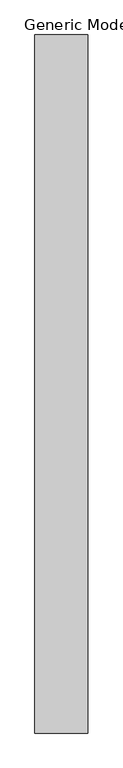
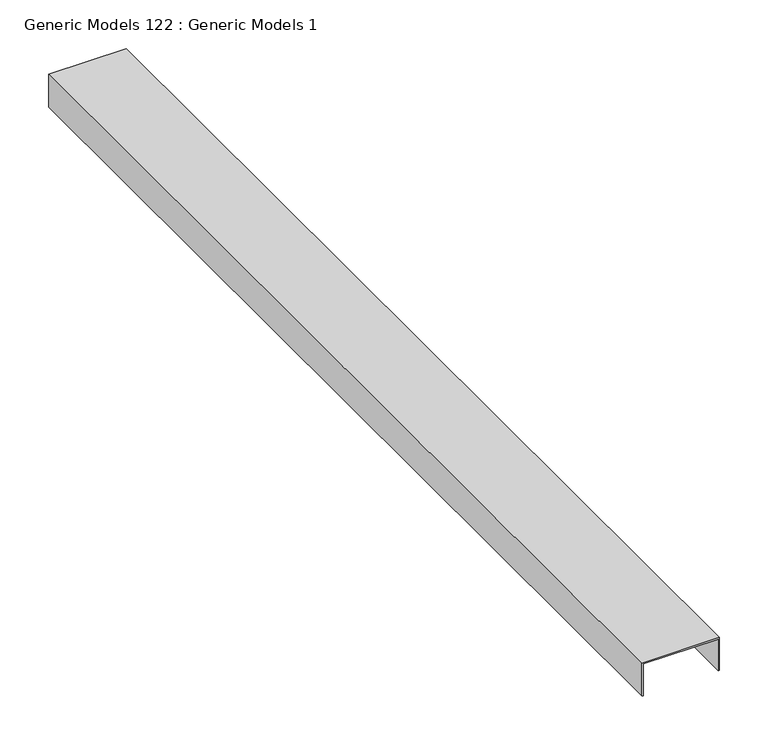
"""IFC4 building model written with IfcOpenShell, lengths in millimetres: proxy geometry, Generic Models 122 : Generic Models 1."""

from ifc_helpers import new_model, si_unit, frame, origin, place, context, project, spatial, polyline, outline, extrude, source, transform, mapped, element, save


def generic_models_122_generic_models_1_f23aae59(model_context):
    return source(origin(), model_context, "Body", "SweptSolid", [
        extrude(outline(polyline([(307.0266124, 49802.3181639), (307.0266124, 49710.2431639), (265.7516124, 49710.2431639), (265.7516124, 49711.8306639), (305.4391124, 49711.8306639), (305.4391124, 49800.7306639), (265.7516124, 49800.7306639), (265.7516124, 49802.3181639), (307.0266124, 49802.3181639)])), frame((0.0, 0.0, 0.0), z_axis=(0.0, 1.0, 0.0), x_axis=(0.0, 0.0, 1.0)), (0.0, 0.0, 1.0), 1219.2),
    ])


if __name__ == "__main__":
    model = new_model("IFC4")
    model_context = context("Model", 3, world=origin())
    ifc_project = project(units=[si_unit("LENGTHUNIT", "METRE", prefix="MILLI")], contexts=[model_context])
    site = spatial("IfcSite", under=ifc_project)
    building = spatial("IfcBuilding", under=site)
    placement = place(None, origin())
    generic_models_122_generic_models_1_shape = generic_models_122_generic_models_1_f23aae59(model_context)
    element("IfcBuildingElementProxy", 1, Name="Generic Models 122 : Generic Models 1", ObjectType="Generic Models 122 : Generic Models 1", at=placement, inside=building, context=model_context, shape_type="MappedRepresentation", body=[
        mapped(generic_models_122_generic_models_1_shape, transform((0.0, 0.0, 0.0), x_axis=(1.0, 0.0, 0.0), y_axis=(0.0, 1.0, 0.0), z_axis=(0.0, 0.0, 1.0))),
    ])
    save(model, "model.ifc")

# Revit data of these elements
# Element 1 (IfcBuildingElementProxy, "Generic Models 122 : Generic Models 1")
#   Materials on its faces: "DEEP LEG OF DEFLECTION TRACK (2\" MIN. DEFLECTION)"
# Materials
#   "DEEP LEG OF DEFLECTION TRACK (2\" MIN. DEFLECTION)": class "Unassigned", colour RGB 210 209 208, transparency 0, Keynote = "M05121300.02", Cost = 0
